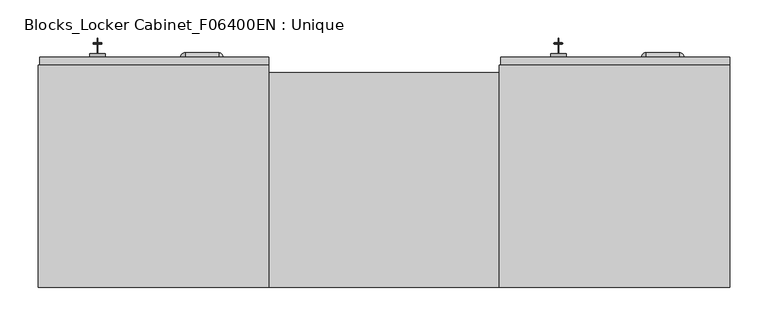
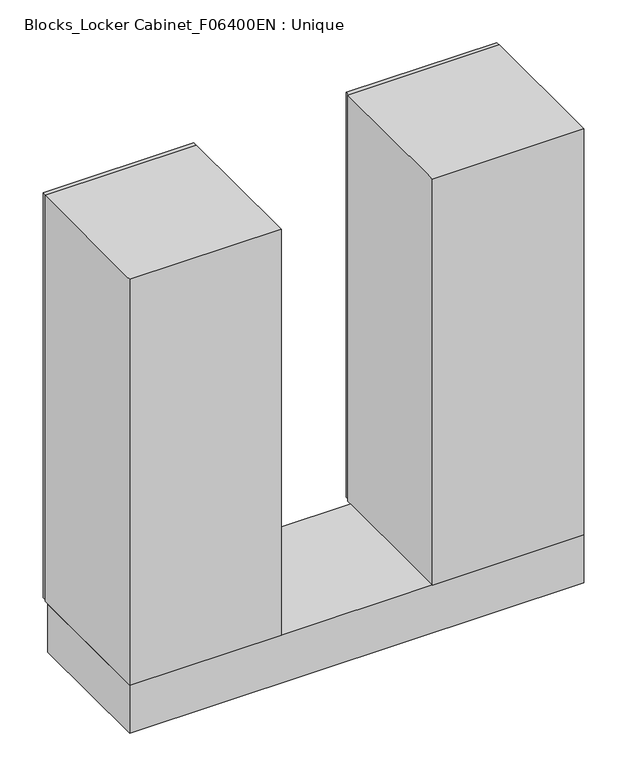
"""IFC4 building model written with IfcOpenShell, lengths in millimetres: furniture geometry, Blocks_Locker Cabinet_F06400EN : Unique."""

from ifc_helpers import new_model, si_unit, point, frame, frame_2d, origin, origin_with_axes, place, context, project, spatial, polyline, circle_curve, ellipse_curve, trimmed, segment, composite_curve, outline, extrude, faceted_brep, source, transform, mapped, element, save
from ifc_brep_helpers import plane_surface, cylinder_surface, revolved_surface, advanced_brep


def blocks_locker_cabinet_f06400en_unique_000e14be(model_context):
    return source(origin(), model_context, "Body", "SolidModel", [
        advanced_brep(
        [(217.0, 12.5, 525.0), (237.0, 12.5, 525.0), (228.8411805, 12.5, 532.0962926), (225.1588195, 12.5, 532.0962926), (225.1588195, 12.5, 522.8618188), (228.8411805, 12.5, 522.8618188), (217.0, 7.5, 525.0), (237.0, 7.5, 525.0), (237.0, 10.7450625, 525.0), (217.0, 10.7450625, 525.0), (228.8411805, 10.7450625, 522.8618188), (228.8411805, 10.7450625, 532.0962926), (225.1588195, 10.7450625, 522.8618188), (225.1588195, 10.7450625, 532.0962926)],
        [
            (0, 1, circle_curve(frame((227.0, 12.5, 525.0), z_axis=(0.0, 1.0, 0.0), x_axis=(1.0, 0.0, 0.0)), 10.0)),
            (1, 0, circle_curve(frame((227.0, 12.5, 525.0), z_axis=(0.0, 1.0, 0.0), x_axis=(1.0, 0.0, 0.0)), 10.0)),
            (2, 3),
            (3, 4),
            (4, 5),
            (5, 2),
            (6, 7, circle_curve(frame((227.0, 7.5, 525.0), z_axis=(0.0, -1.0, 0.0), x_axis=(1.0, 0.0, 0.0)), 10.0)),
            (7, 6, circle_curve(frame((227.0, 7.5, 525.0), z_axis=(0.0, -1.0, 0.0), x_axis=(1.0, 0.0, 0.0)), 10.0)),
            (1, 8),
            (8, 7),
            (6, 9),
            (9, 0),
            (5, 10),
            (10, 11),
            (11, 2),
            (4, 12),
            (12, 10),
            (3, 13),
            (13, 12),
            (11, 13),
        ],
        [
            plane_surface(frame((237.0, 12.5, 525.0), z_axis=(0.0, 1.0, 0.0), x_axis=(0.0, 0.0, 1.0))),
            plane_surface(frame((237.0, 7.5, 525.0), z_axis=(0.0, -1.0, 0.0), x_axis=(0.0, 0.0, -1.0))),
            cylinder_surface(frame((227.0, 7.5, 525.0), z_axis=(0.0, 1.0, 0.0), x_axis=(1.0, 0.0, 0.0)), 10.0),
            plane_surface(frame((228.8411805, 12.5, 532.0962926), z_axis=(-1.0, 0.0, 0.0), x_axis=(0.0, -1.0, 0.0))),
            plane_surface(frame((228.8411805, 12.5, 522.8618188), z_axis=(0.0, 0.0, 1.0), x_axis=(0.0, -1.0, 0.0))),
            plane_surface(frame((225.1588195, 12.5, 522.8618188), z_axis=(1.0, 0.0, 0.0), x_axis=(0.0, -1.0, 0.0))),
            plane_surface(frame((225.1588195, 12.5, 532.0962926), z_axis=(0.0, 0.0, -1.0), x_axis=(0.0, -1.0, 0.0))),
            plane_surface(frame((237.0, 10.7450625, 525.0), z_axis=(0.0, 1.0, 0.0), x_axis=(0.0, 0.0, 1.0))),
        ],
        [
            (0, [[1, 2], [3, 4, 5, 6]]),
            (1, [[7, 8]]),
            (2, [[9, 10, -7, 11, 12, -2]]),
            (2, [[-12, -11, -8, -10, -9, -1]]),
            (3, [[13, 14, 15, -6]]),
            (4, [[16, 17, -13, -5]]),
            (5, [[18, 19, -16, -4]]),
            (6, [[-15, 20, -18, -3]]),
            (7, [[-17, -19, -20, -14]]),
        ],
    ),
        extrude(outline(composite_curve([segment(polyline([(16.8246351, 522.8618188), (13.7848488, 522.8618188)]), True, "CONTINUOUS"), segment(trimmed(circle_curve(frame_2d((12.908516, 522.8618188)), 0.8763328), [point((13.7848488, 522.8618188))], [point((12.0321832, 522.8618188))], True, "CARTESIAN"), True, "CONTINUOUS"), segment(polyline([(12.0321832, 522.8618188), (10.7450625, 522.8618188), (10.7450625, 527.6669902), (17.0336838, 527.6669902)]), True, "CONTINUOUS"), segment(trimmed(circle_curve(frame_2d((23.0067332, 525.0)), 6.5414185), [point((17.0336838, 527.6669902))], [point((16.8246351, 522.8618188))], False, "CARTESIAN"), True, "CONTINUOUS")], self_intersect=False), holes=[composite_curve([segment(trimmed(circle_curve(frame_2d((25.6281997, 525.0)), 1.688217), [point((27.3164167, 525.0))], [point((23.9399827, 525.0))], True, "CARTESIAN"), True, "CONTINUOUS"), segment(trimmed(circle_curve(frame_2d((25.6281997, 525.0)), 1.688217), [point((23.9399827, 525.0))], [point((27.3164167, 525.0))], True, "CARTESIAN"), True, "CONTINUOUS")], self_intersect=False)]), frame((226.5956922, 0.0, 0.0), z_axis=(1.0, 0.0, 0.0), x_axis=(0.0, 1.0, 0.0)), (0.0, 0.0, 1.0), 0.9157402),
        extrude(outline(composite_curve([segment(polyline([(27.8125, 504.8018875), (27.8125, 501.7621012)]), True, "CONTINUOUS"), segment(trimmed(circle_curve(frame_2d((27.8125, 500.8857684)), 0.8763328), [point((27.8125, 501.7621012))], [point((27.8125, 500.0094356))], True, "CARTESIAN"), True, "CONTINUOUS"), segment(polyline([(27.8125, 500.0094356), (27.8125, 497.7621012)]), True, "CONTINUOUS"), segment(trimmed(circle_curve(frame_2d((27.8125, 496.8857684)), 0.8763328), [point((27.8125, 497.7621012))], [point((27.8125, 496.0094356))], True, "CARTESIAN"), True, "CONTINUOUS"), segment(polyline([(27.8125, 496.0094356), (27.8125, 493.7621012)]), True, "CONTINUOUS"), segment(trimmed(circle_curve(frame_2d((27.8125, 492.8857684)), 0.8763328), [point((27.8125, 493.7621012))], [point((27.8125, 492.0094356))], True, "CARTESIAN"), True, "CONTINUOUS"), segment(polyline([(27.8125, 492.0094356), (27.8125, 490.3532579), (25.9613419, 487.7095301), (24.2573286, 487.7095301), (24.2573286, 504.5978839)]), True, "CONTINUOUS"), segment(trimmed(circle_curve(frame_2d((25.6743188, 510.9839856)), 6.5414185), [point((24.2573286, 504.5978839))], [point((27.8125, 504.8018875))], False, "CARTESIAN"), True, "CONTINUOUS")], self_intersect=False), holes=[composite_curve([segment(trimmed(circle_curve(frame_2d((25.6743188, 513.6054521)), 1.688217), [point((25.6743188, 515.2936691))], [point((25.6743188, 511.9172351))], True, "CARTESIAN"), True, "CONTINUOUS"), segment(trimmed(circle_curve(frame_2d((25.6743188, 513.6054521)), 1.688217), [point((25.6743188, 511.9172351))], [point((25.6743188, 515.2936691))], True, "CARTESIAN"), True, "CONTINUOUS")], self_intersect=False)]), frame((226.5956922, 0.0, 0.0), z_axis=(1.0, 0.0, 0.0), x_axis=(0.0, 1.0, 0.0)), (0.0, 0.0, 1.0), 0.9157402),
        advanced_brep(
        [(231.2, 25.663019, 519.4000012), (232.8, 25.663019, 519.4000012), (221.2, 25.663019, 519.4000012), (222.8, 25.663019, 519.4000012)],
        [
            (0, 1, circle_curve(frame((232.0, 25.663019, 519.4000012), z_axis=(0.0, 0.0, -1.0), x_axis=(-1.0, 0.0, 0.0)), 0.8)),
            (1, 2, circle_curve(frame((227.0, 25.663019, 519.4000012), z_axis=(0.0, 1.0, 0.0), x_axis=(-1.0, 0.0, 0.0)), 5.8)),
            (2, 3, circle_curve(frame((222.0, 25.663019, 519.4000012), z_axis=(0.0, 0.0, -1.0), x_axis=(1.0, 0.0, 0.0)), 0.8)),
            (3, 0, circle_curve(frame((227.0, 25.663019, 519.4000012), z_axis=(0.0, -1.0, 0.0), x_axis=(-1.0, 0.0, 0.0)), 4.2)),
            (1, 0, circle_curve(frame((232.0, 25.663019, 519.4000012), z_axis=(0.0, 0.0, -1.0), x_axis=(-1.0, 0.0, 0.0)), 0.8)),
            (3, 2, circle_curve(frame((222.0, 25.663019, 519.4000012), z_axis=(0.0, 0.0, -1.0), x_axis=(1.0, 0.0, 0.0)), 0.8)),
            (2, 1, circle_curve(frame((227.0, 25.663019, 519.4000012), z_axis=(0.0, 1.0, 0.0), x_axis=(1.0, 0.0, 0.0)), 5.8)),
            (0, 3, circle_curve(frame((227.0, 25.663019, 519.4000012), z_axis=(0.0, -1.0, 0.0), x_axis=(1.0, 0.0, 0.0)), 4.2)),
        ],
        [
            revolved_surface(trimmed(ellipse_curve(frame((222.0, 25.663019, 519.4000012), z_axis=(0.0, 0.0, -1.0), x_axis=(1.0, 0.0, 0.0)), 0.8, 0.8), [point((221.2, 25.663019, 519.4000012))], [point((222.8, 25.663019, 519.4000012))], True, "CARTESIAN"), (227.0, -2.5, 519.4000012), (0.0, 1.0, 0.0)),
            revolved_surface(trimmed(ellipse_curve(frame((222.0, 25.663019, 519.4000012), z_axis=(0.0, 0.0, -1.0), x_axis=(1.0, 0.0, 0.0)), 0.8, 0.8), [point((222.8, 25.663019, 519.4000012))], [point((221.2, 25.663019, 519.4000012))], True, "CARTESIAN"), (227.0, -2.5, 519.4000012), (0.0, 1.0, 0.0)),
            revolved_surface(trimmed(ellipse_curve(frame((232.0, 25.663019, 519.4000012), z_axis=(0.0, 0.0, 1.0), x_axis=(-1.0, 0.0, 0.0)), 0.8, 0.8), [point((232.8, 25.663019, 519.4000012))], [point((231.2, 25.663019, 519.4000012))], True, "CARTESIAN"), (227.0, -2.5, 519.4000012), (0.0, 1.0, 0.0)),
            revolved_surface(trimmed(ellipse_curve(frame((232.0, 25.663019, 519.4000012), z_axis=(0.0, 0.0, 1.0), x_axis=(-1.0, 0.0, 0.0)), 0.8, 0.8), [point((231.2, 25.663019, 519.4000012))], [point((232.8, 25.663019, 519.4000012))], True, "CARTESIAN"), (227.0, -2.5, 519.4000012), (0.0, 1.0, 0.0)),
        ],
        [
            (0, [[1, 2, 3, 4]]),
            (1, [[5, -4, 6, -2]]),
            (2, [[-3, 7, -1, 8]]),
            (3, [[-6, -8, -5, -7]]),
        ],
    ),
        advanced_brep(
        [(152.0, 7.5, 949.0), (152.0, -2.5, 949.0), (450.0, -2.5, 949.0), (450.0, 7.5, 949.0), (152.0, 7.5, 101.0), (450.0, 7.5, 101.0), (450.0, -2.5, 101.0), (152.0, -2.5, 101.0), (207.0, 7.5, 675.0), (207.0, 7.5, 555.0), (266.2109264, 7.5, 555.0), (266.2109264, 7.5, 675.0), (219.3473099, 0.3712773, 675.0), (242.7894451, 3.975278, 675.0), (219.3473099, 0.3712773, 555.0), (242.7894451, 3.975278, 555.0)],
        [
            (0, 1),
            (1, 2),
            (2, 3),
            (3, 0),
            (4, 5),
            (5, 6),
            (6, 7),
            (7, 4),
            (3, 5),
            (4, 0),
            (8, 9),
            (9, 10),
            (10, 11),
            (11, 8),
            (2, 6),
            (1, 7),
            (12, 8),
            (11, 13),
            (13, 12, circle_curve(frame((228.8223477, 16.7825242, 675.0), z_axis=(0.0, 0.0, -1.0), x_axis=(0.0, 1.0, 0.0)), 18.9500756)),
            (14, 15, circle_curve(frame((228.8223477, 16.7825242, 555.0), z_axis=(0.0, 0.0, 1.0), x_axis=(0.0, 1.0, 0.0)), 18.9500756)),
            (15, 10),
            (9, 14),
            (12, 14),
            (15, 13),
        ],
        [
            plane_surface(frame((450.0, 7.5, 949.0), z_axis=(0.0, 0.0, 1.0), x_axis=(1.0, 0.0, 0.0))),
            plane_surface(frame((450.0, 7.5, 101.0), z_axis=(0.0, 0.0, -1.0), x_axis=(-1.0, 0.0, 0.0))),
            plane_surface(frame((152.0, 7.5, 949.0), z_axis=(0.0, 1.0, 0.0), x_axis=(0.0, 0.0, -1.0))),
            plane_surface(frame((450.0, 7.5, 949.0), z_axis=(1.0, 0.0, 0.0), x_axis=(0.0, 0.0, -1.0))),
            plane_surface(frame((450.0, -2.5, 949.0), z_axis=(0.0, -1.0, 0.0), x_axis=(0.0, 0.0, -1.0))),
            plane_surface(frame((152.0, -2.5, 949.0), z_axis=(-1.0, 0.0, 0.0), x_axis=(0.0, 0.0, -1.0))),
            plane_surface(frame((207.0, 7.5, 675.0), z_axis=(0.0, 0.0, -1.0), x_axis=(-0.866025403784437, 0.5000000000000028, 0.0))),
            plane_surface(frame((207.0, 7.5, 555.0), z_axis=(0.0, 0.0, 1.0), x_axis=(0.866025403784437, -0.5000000000000028, 0.0))),
            plane_surface(frame((219.3473099, 0.3712773, 675.0), z_axis=(0.5000000000000028, 0.866025403784437, 0.0), x_axis=(0.0, 0.0, -1.0))),
            plane_surface(frame((266.2109264, 7.5, 675.0), z_axis=(-0.14881527984319862, 0.9888650122666847, 0.0), x_axis=(0.0, 0.0, -1.0))),
            revolved_surface(polyline([(228.8223477, 35.7325998, 675.0), (228.8223477, 35.7325998, 555.0)]), (228.8223477, 16.7825242, 555.0), (0.0, 0.0, 1.0)),
        ],
        [
            (0, [[1, 2, 3, 4]]),
            (1, [[5, 6, 7, 8]]),
            (2, [[9, -5, 10, -4], [11, 12, 13, 14]]),
            (3, [[15, -6, -9, -3]]),
            (4, [[16, -7, -15, -2]]),
            (5, [[-10, -8, -16, -1]]),
            (6, [[17, -14, 18, 19]]),
            (7, [[20, 21, -12, 22]]),
            (8, [[23, -22, -11, -17]]),
            (9, [[-13, -21, 24, -18]]),
            (10, [[-24, -20, -23, -19]]),
        ],
    ),
        advanced_brep(
        [(335.0, 7.5, 141.0), (390.5189667, 7.5, 141.0), (384.5189667, 7.5, 147.0), (341.0, 7.5, 147.0), (341.0, 13.5, 141.0), (384.5189667, 13.5, 141.0)],
        [
            (0, 1),
            (1, 2, circle_curve(frame((384.5189667, 7.5, 141.0), z_axis=(0.0, -1.0, 0.0), x_axis=(1.0, 0.0, 0.0)), 6.0)),
            (2, 3),
            (3, 0, circle_curve(frame((341.0, 7.5, 141.0), z_axis=(0.0, -1.0, 0.0), x_axis=(1.0, 0.0, 0.0)), 6.0)),
            (0, 4, circle_curve(frame((341.0, 7.5, 141.0), z_axis=(0.0, 0.0, -1.0), x_axis=(1.0, 0.0, 0.0)), 6.0)),
            (4, 5),
            (5, 1, circle_curve(frame((384.5189667, 7.5, 141.0), z_axis=(0.0, 0.0, -1.0), x_axis=(1.0, 0.0, 0.0)), 6.0)),
            (3, 4, circle_curve(frame((341.0, 7.5, 141.0), z_axis=(-1.0, 0.0, 0.0), x_axis=(0.0, 0.0, 1.0)), 6.0)),
            (2, 5, circle_curve(frame((384.5189667, 7.5, 141.0), z_axis=(-1.0, 0.0, 0.0), x_axis=(0.0, 0.0, 1.0)), 6.0)),
        ],
        [
            plane_surface(frame((385.0, 7.5, 141.0), z_axis=(0.0, -1.0, 0.0), x_axis=(0.0, 0.0, 1.0))),
            plane_surface(frame((385.0, 7.5, 141.0), z_axis=(0.0, 0.0, -1.0), x_axis=(0.0, 1.0, 0.0))),
            revolved_surface(trimmed(ellipse_curve(frame((341.0, 7.5, 141.0), z_axis=(0.0, 1.0, 0.0), x_axis=(1.0, 0.0, 0.0)), 6.0, 6.0), [point((335.0, 7.5, 141.0))], [point((341.0, 7.5, 147.0))], True, "CARTESIAN"), (385.0, 7.5, 141.0), (1.0, 0.0, 0.0)),
            cylinder_surface(frame((385.0, 7.5, 141.0), z_axis=(1.0, 0.0, 0.0), x_axis=(0.0, 0.0, 1.0)), 6.0),
            revolved_surface(trimmed(ellipse_curve(frame((384.5189667, 7.5, 141.0), z_axis=(0.0, 1.0, 0.0), x_axis=(1.0, 0.0, 0.0)), 6.0, 6.0), [point((384.5189667, 7.5, 147.0))], [point((390.5189667, 7.5, 141.0))], True, "CARTESIAN"), (385.0, 7.5, 141.0), (1.0, 0.0, 0.0)),
        ],
        [
            (0, [[1, 2, 3, 4]]),
            (1, [[-1, 5, 6, 7]]),
            (2, [[-5, -4, 8]]),
            (3, [[-6, -8, -3, 9]]),
            (4, [[-7, -9, -2]]),
        ],
    ),
        advanced_brep(
        [(335.0, 7.5, 156.0), (390.5189667, 7.5, 156.0), (384.5189667, 7.5, 162.0), (341.0, 7.5, 162.0), (341.0, 13.5, 156.0), (384.5189667, 13.5, 156.0)],
        [
            (0, 1),
            (1, 2, circle_curve(frame((384.5189667, 7.5, 156.0), z_axis=(0.0, -1.0, 0.0), x_axis=(1.0, 0.0, 0.0)), 6.0)),
            (2, 3),
            (3, 0, circle_curve(frame((341.0, 7.5, 156.0), z_axis=(0.0, -1.0, 0.0), x_axis=(1.0, 0.0, 0.0)), 6.0)),
            (0, 4, circle_curve(frame((341.0, 7.5, 156.0), z_axis=(0.0, 0.0, -1.0), x_axis=(1.0, 0.0, 0.0)), 6.0)),
            (4, 5),
            (5, 1, circle_curve(frame((384.5189667, 7.5, 156.0), z_axis=(0.0, 0.0, -1.0), x_axis=(1.0, 0.0, 0.0)), 6.0)),
            (3, 4, circle_curve(frame((341.0, 7.5, 156.0), z_axis=(-1.0, 0.0, 0.0), x_axis=(0.0, 0.0, 1.0)), 6.0)),
            (2, 5, circle_curve(frame((384.5189667, 7.5, 156.0), z_axis=(-1.0, 0.0, 0.0), x_axis=(0.0, 0.0, 1.0)), 6.0)),
        ],
        [
            plane_surface(frame((385.0, 7.5, 156.0), z_axis=(0.0, -1.0, 0.0), x_axis=(0.0, 0.0, 1.0))),
            plane_surface(frame((385.0, 7.5, 156.0), z_axis=(0.0, 0.0, -1.0), x_axis=(0.0, 1.0, 0.0))),
            revolved_surface(trimmed(ellipse_curve(frame((341.0, 7.5, 156.0), z_axis=(0.0, 1.0, 0.0), x_axis=(1.0, 0.0, 0.0)), 6.0, 6.0), [point((335.0, 7.5, 156.0))], [point((341.0, 7.5, 162.0))], True, "CARTESIAN"), (385.0, 7.5, 156.0), (1.0, 0.0, 0.0)),
            cylinder_surface(frame((385.0, 7.5, 156.0), z_axis=(1.0, 0.0, 0.0), x_axis=(0.0, 0.0, 1.0)), 6.0),
            revolved_surface(trimmed(ellipse_curve(frame((384.5189667, 7.5, 156.0), z_axis=(0.0, 1.0, 0.0), x_axis=(1.0, 0.0, 0.0)), 6.0, 6.0), [point((384.5189667, 7.5, 162.0))], [point((390.5189667, 7.5, 156.0))], True, "CARTESIAN"), (385.0, 7.5, 156.0), (1.0, 0.0, 0.0)),
        ],
        [
            (0, [[1, 2, 3, 4]]),
            (1, [[-1, 5, 6, 7]]),
            (2, [[-5, -4, 8]]),
            (3, [[-6, -8, -3, 9]]),
            (4, [[-7, -9, -2]]),
        ],
    ),
        advanced_brep(
        [(335.0, 7.5, 171.0), (390.5189667, 7.5, 171.0), (384.5189667, 7.5, 177.0), (341.0, 7.5, 177.0), (341.0, 13.5, 171.0), (384.5189667, 13.5, 171.0)],
        [
            (0, 1),
            (1, 2, circle_curve(frame((384.5189667, 7.5, 171.0), z_axis=(0.0, -1.0, 0.0), x_axis=(1.0, 0.0, 0.0)), 6.0)),
            (2, 3),
            (3, 0, circle_curve(frame((341.0, 7.5, 171.0), z_axis=(0.0, -1.0, 0.0), x_axis=(1.0, 0.0, 0.0)), 6.0)),
            (0, 4, circle_curve(frame((341.0, 7.5, 171.0), z_axis=(0.0, 0.0, -1.0), x_axis=(1.0, 0.0, 0.0)), 6.0)),
            (4, 5),
            (5, 1, circle_curve(frame((384.5189667, 7.5, 171.0), z_axis=(0.0, 0.0, -1.0), x_axis=(1.0, 0.0, 0.0)), 6.0)),
            (3, 4, circle_curve(frame((341.0, 7.5, 171.0), z_axis=(-1.0, 0.0, 0.0), x_axis=(0.0, 0.0, 1.0)), 6.0)),
            (2, 5, circle_curve(frame((384.5189667, 7.5, 171.0), z_axis=(-1.0, 0.0, 0.0), x_axis=(0.0, 0.0, 1.0)), 6.0)),
        ],
        [
            plane_surface(frame((385.0, 7.5, 171.0), z_axis=(0.0, -1.0, 0.0), x_axis=(0.0, 0.0, 1.0))),
            plane_surface(frame((385.0, 7.5, 171.0), z_axis=(0.0, 0.0, -1.0), x_axis=(0.0, 1.0, 0.0))),
            revolved_surface(trimmed(ellipse_curve(frame((341.0, 7.5, 171.0), z_axis=(0.0, 1.0, 0.0), x_axis=(1.0, 0.0, 0.0)), 6.0, 6.0), [point((335.0, 7.5, 171.0))], [point((341.0, 7.5, 177.0))], True, "CARTESIAN"), (385.0, 7.5, 171.0), (1.0, 0.0, 0.0)),
            cylinder_surface(frame((385.0, 7.5, 171.0), z_axis=(1.0, 0.0, 0.0), x_axis=(0.0, 0.0, 1.0)), 6.0),
            revolved_surface(trimmed(ellipse_curve(frame((384.5189667, 7.5, 171.0), z_axis=(0.0, 1.0, 0.0), x_axis=(1.0, 0.0, 0.0)), 6.0, 6.0), [point((384.5189667, 7.5, 177.0))], [point((390.5189667, 7.5, 171.0))], True, "CARTESIAN"), (385.0, 7.5, 171.0), (1.0, 0.0, 0.0)),
        ],
        [
            (0, [[1, 2, 3, 4]]),
            (1, [[-1, 5, 6, 7]]),
            (2, [[-5, -4, 8]]),
            (3, [[-6, -8, -3, 9]]),
            (4, [[-7, -9, -2]]),
        ],
    ),
        advanced_brep(
        [(335.0, 7.5, 186.0), (390.5189667, 7.5, 186.0), (384.5189667, 7.5, 192.0), (341.0, 7.5, 192.0), (341.0, 13.5, 186.0), (384.5189667, 13.5, 186.0)],
        [
            (0, 1),
            (1, 2, circle_curve(frame((384.5189667, 7.5, 186.0), z_axis=(0.0, -1.0, 0.0), x_axis=(1.0, 0.0, 0.0)), 6.0)),
            (2, 3),
            (3, 0, circle_curve(frame((341.0, 7.5, 186.0), z_axis=(0.0, -1.0, 0.0), x_axis=(1.0, 0.0, 0.0)), 6.0)),
            (0, 4, circle_curve(frame((341.0, 7.5, 186.0), z_axis=(0.0, 0.0, -1.0), x_axis=(1.0, 0.0, 0.0)), 6.0)),
            (4, 5),
            (5, 1, circle_curve(frame((384.5189667, 7.5, 186.0), z_axis=(0.0, 0.0, -1.0), x_axis=(1.0, 0.0, 0.0)), 6.0)),
            (3, 4, circle_curve(frame((341.0, 7.5, 186.0), z_axis=(-1.0, 0.0, 0.0), x_axis=(0.0, 0.0, 1.0)), 6.0)),
            (2, 5, circle_curve(frame((384.5189667, 7.5, 186.0), z_axis=(-1.0, 0.0, 0.0), x_axis=(0.0, 0.0, 1.0)), 6.0)),
        ],
        [
            plane_surface(frame((385.0, 7.5, 186.0), z_axis=(0.0, -1.0, 0.0), x_axis=(0.0, 0.0, 1.0))),
            plane_surface(frame((385.0, 7.5, 186.0), z_axis=(0.0, 0.0, -1.0), x_axis=(0.0, 1.0, 0.0))),
            revolved_surface(trimmed(ellipse_curve(frame((341.0, 7.5, 186.0), z_axis=(0.0, 1.0, 0.0), x_axis=(1.0, 0.0, 0.0)), 6.0, 6.0), [point((335.0, 7.5, 186.0))], [point((341.0, 7.5, 192.0))], True, "CARTESIAN"), (385.0, 7.5, 186.0), (1.0, 0.0, 0.0)),
            cylinder_surface(frame((385.0, 7.5, 186.0), z_axis=(1.0, 0.0, 0.0), x_axis=(0.0, 0.0, 1.0)), 6.0),
            revolved_surface(trimmed(ellipse_curve(frame((384.5189667, 7.5, 186.0), z_axis=(0.0, 1.0, 0.0), x_axis=(1.0, 0.0, 0.0)), 6.0, 6.0), [point((384.5189667, 7.5, 192.0))], [point((390.5189667, 7.5, 186.0))], True, "CARTESIAN"), (385.0, 7.5, 186.0), (1.0, 0.0, 0.0)),
        ],
        [
            (0, [[1, 2, 3, 4]]),
            (1, [[-1, 5, 6, 7]]),
            (2, [[-5, -4, 8]]),
            (3, [[-6, -8, -3, 9]]),
            (4, [[-7, -9, -2]]),
        ],
    ),
        advanced_brep(
        [(335.0, 7.5, 201.0), (390.5189667, 7.5, 201.0), (384.5189667, 7.5, 207.0), (341.0, 7.5, 207.0), (341.0, 13.5, 201.0), (384.5189667, 13.5, 201.0)],
        [
            (0, 1),
            (1, 2, circle_curve(frame((384.5189667, 7.5, 201.0), z_axis=(0.0, -1.0, 0.0), x_axis=(1.0, 0.0, 0.0)), 6.0)),
            (2, 3),
            (3, 0, circle_curve(frame((341.0, 7.5, 201.0), z_axis=(0.0, -1.0, 0.0), x_axis=(1.0, 0.0, 0.0)), 6.0)),
            (0, 4, circle_curve(frame((341.0, 7.5, 201.0), z_axis=(0.0, 0.0, -1.0), x_axis=(1.0, 0.0, 0.0)), 6.0)),
            (4, 5),
            (5, 1, circle_curve(frame((384.5189667, 7.5, 201.0), z_axis=(0.0, 0.0, -1.0), x_axis=(1.0, 0.0, 0.0)), 6.0)),
            (3, 4, circle_curve(frame((341.0, 7.5, 201.0), z_axis=(-1.0, 0.0, 0.0), x_axis=(0.0, 0.0, 1.0)), 6.0)),
            (2, 5, circle_curve(frame((384.5189667, 7.5, 201.0), z_axis=(-1.0, 0.0, 0.0), x_axis=(0.0, 0.0, 1.0)), 6.0)),
        ],
        [
            plane_surface(frame((385.0, 7.5, 201.0), z_axis=(0.0, -1.0, 0.0), x_axis=(0.0, 0.0, 1.0))),
            plane_surface(frame((385.0, 7.5, 201.0), z_axis=(0.0, 0.0, -1.0), x_axis=(0.0, 1.0, 0.0))),
            revolved_surface(trimmed(ellipse_curve(frame((341.0, 7.5, 201.0), z_axis=(0.0, 1.0, 0.0), x_axis=(1.0, 0.0, 0.0)), 6.0, 6.0), [point((335.0, 7.5, 201.0))], [point((341.0, 7.5, 207.0))], True, "CARTESIAN"), (385.0, 7.5, 201.0), (1.0, 0.0, 0.0)),
            cylinder_surface(frame((385.0, 7.5, 201.0), z_axis=(1.0, 0.0, 0.0), x_axis=(0.0, 0.0, 1.0)), 6.0),
            revolved_surface(trimmed(ellipse_curve(frame((384.5189667, 7.5, 201.0), z_axis=(0.0, 1.0, 0.0), x_axis=(1.0, 0.0, 0.0)), 6.0, 6.0), [point((384.5189667, 7.5, 207.0))], [point((390.5189667, 7.5, 201.0))], True, "CARTESIAN"), (385.0, 7.5, 201.0), (1.0, 0.0, 0.0)),
        ],
        [
            (0, [[1, 2, 3, 4]]),
            (1, [[-1, 5, 6, 7]]),
            (2, [[-5, -4, 8]]),
            (3, [[-6, -8, -3, 9]]),
            (4, [[-7, -9, -2]]),
        ],
    ),
        extrude(outline(composite_curve([segment(polyline([(219.3473099, 0.3712773), (207.0, 7.5), (266.2109264, 7.5), (242.7894451, 3.975278)]), True, "CONTINUOUS"), segment(trimmed(circle_curve(frame_2d((228.8223477, 16.7825242)), 18.9500756), [point((242.7894451, 3.975278))], [point((219.3473099, 0.3712773))], False, "CARTESIAN"), True, "CONTINUOUS")], self_intersect=False)), frame((0.0, 0.0, 555.0), z_axis=(0.0, 0.0, 1.0), x_axis=(1.0, 0.0, 0.0)), (0.0, 0.0, 1.0), 5.0),
        extrude(outline(composite_curve([segment(polyline([(219.3473099, 0.3712773), (207.0, 7.5), (266.2109264, 7.5), (242.7894451, 3.975278)]), True, "CONTINUOUS"), segment(trimmed(circle_curve(frame_2d((228.8223477, 16.7825242)), 18.9500756), [point((242.7894451, 3.975278))], [point((219.3473099, 0.3712773))], False, "CARTESIAN"), True, "CONTINUOUS")], self_intersect=False)), frame((0.0, 0.0, 670.0), z_axis=(0.0, 0.0, 1.0), x_axis=(1.0, 0.0, 0.0)), (0.0, 0.0, 1.0), 5.0),
        faceted_brep([(450.0, -2.5, 950.0), (450.0, -2.5, 100.0), (150.0, -2.5, 100.0), (150.0, -2.5, 950.0), (440.0, -2.5, 940.0), (160.0, -2.5, 940.0), (160.0, -2.5, 110.0), (440.0, -2.5, 110.0), (450.0, -292.5, 950.0), (150.0, -292.5, 950.0), (150.0, -292.5, 100.0), (450.0, -292.5, 100.0), (150.0, -282.5, 950.0), (450.0, -282.5, 950.0), (150.0, -282.5, 100.0), (450.0, -282.5, 100.0), (440.0, -282.5, 110.0), (440.0, -282.5, 940.0), (160.0, -282.5, 110.0), (160.0, -282.5, 940.0)], [[[0, 1, 2, 3], [4, 5, 6, 7]], [[8, 9, 10, 11]], [[3, 12, 9, 8, 13, 0]], [[2, 14, 10, 9, 12, 3]], [[1, 15, 11, 10, 14, 2]], [[0, 13, 8, 11, 15, 1]], [[7, 16, 17, 4]], [[6, 18, 16, 7]], [[5, 19, 18, 6]], [[4, 17, 19, 5]], [[16, 18, 19, 17]]]),
        advanced_brep(
        [(-383.0, 12.5, 525.0), (-363.0, 12.5, 525.0), (-371.1588195, 12.5, 532.0962926), (-374.8411805, 12.5, 532.0962926), (-374.8411805, 12.5, 522.8618188), (-371.1588195, 12.5, 522.8618188), (-383.0, 7.5, 525.0), (-363.0, 7.5, 525.0), (-363.0, 10.7450625, 525.0), (-383.0, 10.7450625, 525.0), (-371.1588195, 10.7450625, 522.8618188), (-371.1588195, 10.7450625, 532.0962926), (-374.8411805, 10.7450625, 522.8618188), (-374.8411805, 10.7450625, 532.0962926)],
        [
            (0, 1, circle_curve(frame((-373.0, 12.5, 525.0), z_axis=(0.0, 1.0, 0.0), x_axis=(1.0, 0.0, 0.0)), 10.0)),
            (1, 0, circle_curve(frame((-373.0, 12.5, 525.0), z_axis=(0.0, 1.0, 0.0), x_axis=(1.0, 0.0, 0.0)), 10.0)),
            (2, 3),
            (3, 4),
            (4, 5),
            (5, 2),
            (6, 7, circle_curve(frame((-373.0, 7.5, 525.0), z_axis=(0.0, -1.0, 0.0), x_axis=(1.0, 0.0, 0.0)), 10.0)),
            (7, 6, circle_curve(frame((-373.0, 7.5, 525.0), z_axis=(0.0, -1.0, 0.0), x_axis=(1.0, 0.0, 0.0)), 10.0)),
            (1, 8),
            (8, 7),
            (6, 9),
            (9, 0),
            (5, 10),
            (10, 11),
            (11, 2),
            (4, 12),
            (12, 10),
            (3, 13),
            (13, 12),
            (11, 13),
        ],
        [
            plane_surface(frame((-363.0, 12.5, 525.0), z_axis=(0.0, 1.0, 0.0), x_axis=(0.0, 0.0, 1.0))),
            plane_surface(frame((-363.0, 7.5, 525.0), z_axis=(0.0, -1.0, 0.0), x_axis=(0.0, 0.0, -1.0))),
            cylinder_surface(frame((-373.0, 7.5, 525.0), z_axis=(0.0, 1.0, 0.0), x_axis=(1.0, 0.0, 0.0)), 10.0),
            plane_surface(frame((-371.1588195, 12.5, 532.0962926), z_axis=(-1.0, 0.0, 0.0), x_axis=(0.0, -1.0, 0.0))),
            plane_surface(frame((-371.1588195, 12.5, 522.8618188), z_axis=(0.0, 0.0, 1.0), x_axis=(0.0, -1.0, 0.0))),
            plane_surface(frame((-374.8411805, 12.5, 522.8618188), z_axis=(1.0, 0.0, 0.0), x_axis=(0.0, -1.0, 0.0))),
            plane_surface(frame((-374.8411805, 12.5, 532.0962926), z_axis=(0.0, 0.0, -1.0), x_axis=(0.0, -1.0, 0.0))),
            plane_surface(frame((-363.0, 10.7450625, 525.0), z_axis=(0.0, 1.0, 0.0), x_axis=(0.0, 0.0, 1.0))),
        ],
        [
            (0, [[1, 2], [3, 4, 5, 6]]),
            (1, [[7, 8]]),
            (2, [[9, 10, -7, 11, 12, -2]]),
            (2, [[-12, -11, -8, -10, -9, -1]]),
            (3, [[13, 14, 15, -6]]),
            (4, [[16, 17, -13, -5]]),
            (5, [[18, 19, -16, -4]]),
            (6, [[-15, 20, -18, -3]]),
            (7, [[-17, -19, -20, -14]]),
        ],
    ),
        extrude(outline(composite_curve([segment(polyline([(16.8246351, 522.8618188), (13.7848488, 522.8618188)]), True, "CONTINUOUS"), segment(trimmed(circle_curve(frame_2d((12.908516, 522.8618188)), 0.8763328), [point((13.7848488, 522.8618188))], [point((12.0321832, 522.8618188))], True, "CARTESIAN"), True, "CONTINUOUS"), segment(polyline([(12.0321832, 522.8618188), (10.7450625, 522.8618188), (10.7450625, 527.6669902), (17.0336838, 527.6669902)]), True, "CONTINUOUS"), segment(trimmed(circle_curve(frame_2d((23.0067332, 525.0)), 6.5414185), [point((17.0336838, 527.6669902))], [point((16.8246351, 522.8618188))], False, "CARTESIAN"), True, "CONTINUOUS")], self_intersect=False), holes=[composite_curve([segment(trimmed(circle_curve(frame_2d((25.6281997, 525.0)), 1.688217), [point((27.3164167, 525.0))], [point((23.9399827, 525.0))], True, "CARTESIAN"), True, "CONTINUOUS"), segment(trimmed(circle_curve(frame_2d((25.6281997, 525.0)), 1.688217), [point((23.9399827, 525.0))], [point((27.3164167, 525.0))], True, "CARTESIAN"), True, "CONTINUOUS")], self_intersect=False)]), frame((-373.4043078, 0.0, 0.0), z_axis=(1.0, 0.0, 0.0), x_axis=(0.0, 1.0, 0.0)), (0.0, 0.0, 1.0), 0.9157402),
        extrude(outline(composite_curve([segment(polyline([(27.8125, 504.8018875), (27.8125, 501.7621012)]), True, "CONTINUOUS"), segment(trimmed(circle_curve(frame_2d((27.8125, 500.8857684)), 0.8763328), [point((27.8125, 501.7621012))], [point((27.8125, 500.0094356))], True, "CARTESIAN"), True, "CONTINUOUS"), segment(polyline([(27.8125, 500.0094356), (27.8125, 497.7621012)]), True, "CONTINUOUS"), segment(trimmed(circle_curve(frame_2d((27.8125, 496.8857684)), 0.8763328), [point((27.8125, 497.7621012))], [point((27.8125, 496.0094356))], True, "CARTESIAN"), True, "CONTINUOUS"), segment(polyline([(27.8125, 496.0094356), (27.8125, 493.7621012)]), True, "CONTINUOUS"), segment(trimmed(circle_curve(frame_2d((27.8125, 492.8857684)), 0.8763328), [point((27.8125, 493.7621012))], [point((27.8125, 492.0094356))], True, "CARTESIAN"), True, "CONTINUOUS"), segment(polyline([(27.8125, 492.0094356), (27.8125, 490.3532579), (25.9613419, 487.7095301), (24.2573286, 487.7095301), (24.2573286, 504.5978839)]), True, "CONTINUOUS"), segment(trimmed(circle_curve(frame_2d((25.6743188, 510.9839856)), 6.5414185), [point((24.2573286, 504.5978839))], [point((27.8125, 504.8018875))], False, "CARTESIAN"), True, "CONTINUOUS")], self_intersect=False), holes=[composite_curve([segment(trimmed(circle_curve(frame_2d((25.6743188, 513.6054521)), 1.688217), [point((25.6743188, 515.2936691))], [point((25.6743188, 511.9172351))], True, "CARTESIAN"), True, "CONTINUOUS"), segment(trimmed(circle_curve(frame_2d((25.6743188, 513.6054521)), 1.688217), [point((25.6743188, 511.9172351))], [point((25.6743188, 515.2936691))], True, "CARTESIAN"), True, "CONTINUOUS")], self_intersect=False)]), frame((-373.4043078, 0.0, 0.0), z_axis=(1.0, 0.0, 0.0), x_axis=(0.0, 1.0, 0.0)), (0.0, 0.0, 1.0), 0.9157402),
        advanced_brep(
        [(-368.8, 25.663019, 519.4000012), (-367.2, 25.663019, 519.4000012), (-378.8, 25.663019, 519.4000012), (-377.2, 25.663019, 519.4000012)],
        [
            (0, 1, circle_curve(frame((-368.0, 25.663019, 519.4000012), z_axis=(0.0, 0.0, -1.0), x_axis=(-1.0, 0.0, 0.0)), 0.8)),
            (1, 2, circle_curve(frame((-373.0, 25.663019, 519.4000012), z_axis=(0.0, 1.0, 0.0), x_axis=(-1.0, 0.0, 0.0)), 5.8)),
            (2, 3, circle_curve(frame((-378.0, 25.663019, 519.4000012), z_axis=(0.0, 0.0, -1.0), x_axis=(1.0, 0.0, 0.0)), 0.8)),
            (3, 0, circle_curve(frame((-373.0, 25.663019, 519.4000012), z_axis=(0.0, -1.0, 0.0), x_axis=(-1.0, 0.0, 0.0)), 4.2)),
            (1, 0, circle_curve(frame((-368.0, 25.663019, 519.4000012), z_axis=(0.0, 0.0, -1.0), x_axis=(-1.0, 0.0, 0.0)), 0.8)),
            (3, 2, circle_curve(frame((-378.0, 25.663019, 519.4000012), z_axis=(0.0, 0.0, -1.0), x_axis=(1.0, 0.0, 0.0)), 0.8)),
            (2, 1, circle_curve(frame((-373.0, 25.663019, 519.4000012), z_axis=(0.0, 1.0, 0.0), x_axis=(1.0, 0.0, 0.0)), 5.8)),
            (0, 3, circle_curve(frame((-373.0, 25.663019, 519.4000012), z_axis=(0.0, -1.0, 0.0), x_axis=(1.0, 0.0, 0.0)), 4.2)),
        ],
        [
            revolved_surface(trimmed(ellipse_curve(frame((-378.0, 25.663019, 519.4000012), z_axis=(0.0, 0.0, -1.0), x_axis=(1.0, 0.0, 0.0)), 0.8, 0.8), [point((-378.8, 25.663019, 519.4000012))], [point((-377.2, 25.663019, 519.4000012))], True, "CARTESIAN"), (-373.0, -2.5, 519.4000012), (0.0, 1.0, 0.0)),
            revolved_surface(trimmed(ellipse_curve(frame((-378.0, 25.663019, 519.4000012), z_axis=(0.0, 0.0, -1.0), x_axis=(1.0, 0.0, 0.0)), 0.8, 0.8), [point((-377.2, 25.663019, 519.4000012))], [point((-378.8, 25.663019, 519.4000012))], True, "CARTESIAN"), (-373.0, -2.5, 519.4000012), (0.0, 1.0, 0.0)),
            revolved_surface(trimmed(ellipse_curve(frame((-368.0, 25.663019, 519.4000012), z_axis=(0.0, 0.0, 1.0), x_axis=(-1.0, 0.0, 0.0)), 0.8, 0.8), [point((-367.2, 25.663019, 519.4000012))], [point((-368.8, 25.663019, 519.4000012))], True, "CARTESIAN"), (-373.0, -2.5, 519.4000012), (0.0, 1.0, 0.0)),
            revolved_surface(trimmed(ellipse_curve(frame((-368.0, 25.663019, 519.4000012), z_axis=(0.0, 0.0, 1.0), x_axis=(-1.0, 0.0, 0.0)), 0.8, 0.8), [point((-368.8, 25.663019, 519.4000012))], [point((-367.2, 25.663019, 519.4000012))], True, "CARTESIAN"), (-373.0, -2.5, 519.4000012), (0.0, 1.0, 0.0)),
        ],
        [
            (0, [[1, 2, 3, 4]]),
            (1, [[5, -4, 6, -2]]),
            (2, [[-3, 7, -1, 8]]),
            (3, [[-6, -8, -5, -7]]),
        ],
    ),
        advanced_brep(
        [(-448.0, 7.5, 949.0), (-448.0, -2.5, 949.0), (-150.0, -2.5, 949.0), (-150.0, 7.5, 949.0), (-448.0, 7.5, 101.0), (-150.0, 7.5, 101.0), (-150.0, -2.5, 101.0), (-448.0, -2.5, 101.0), (-393.0, 7.5, 675.0), (-393.0, 7.5, 555.0), (-333.7890736, 7.5, 555.0), (-333.7890736, 7.5, 675.0), (-380.6526901, 0.3712773, 675.0), (-357.2105549, 3.975278, 675.0), (-380.6526901, 0.3712773, 555.0), (-357.2105549, 3.975278, 555.0)],
        [
            (0, 1),
            (1, 2),
            (2, 3),
            (3, 0),
            (4, 5),
            (5, 6),
            (6, 7),
            (7, 4),
            (3, 5),
            (4, 0),
            (8, 9),
            (9, 10),
            (10, 11),
            (11, 8),
            (2, 6),
            (1, 7),
            (12, 8),
            (11, 13),
            (13, 12, circle_curve(frame((-371.1776523, 16.7825242, 675.0), z_axis=(0.0, 0.0, -1.0), x_axis=(0.0, 1.0, 0.0)), 18.9500756)),
            (14, 15, circle_curve(frame((-371.1776523, 16.7825242, 555.0), z_axis=(0.0, 0.0, 1.0), x_axis=(0.0, 1.0, 0.0)), 18.9500756)),
            (15, 10),
            (9, 14),
            (12, 14),
            (15, 13),
        ],
        [
            plane_surface(frame((-150.0, 7.5, 949.0), z_axis=(0.0, 0.0, 1.0), x_axis=(1.0, 0.0, 0.0))),
            plane_surface(frame((-150.0, 7.5, 101.0), z_axis=(0.0, 0.0, -1.0), x_axis=(-1.0, 0.0, 0.0))),
            plane_surface(frame((-448.0, 7.5, 949.0), z_axis=(0.0, 1.0, 0.0), x_axis=(0.0, 0.0, -1.0))),
            plane_surface(frame((-150.0, 7.5, 949.0), z_axis=(1.0, 0.0, 0.0), x_axis=(0.0, 0.0, -1.0))),
            plane_surface(frame((-150.0, -2.5, 949.0), z_axis=(0.0, -1.0, 0.0), x_axis=(0.0, 0.0, -1.0))),
            plane_surface(frame((-448.0, -2.5, 949.0), z_axis=(-1.0, 0.0, 0.0), x_axis=(0.0, 0.0, -1.0))),
            plane_surface(frame((-393.0, 7.5, 675.0), z_axis=(0.0, 0.0, -1.0), x_axis=(-0.866025403784437, 0.5000000000000028, 0.0))),
            plane_surface(frame((-393.0, 7.5, 555.0), z_axis=(0.0, 0.0, 1.0), x_axis=(0.866025403784437, -0.5000000000000028, 0.0))),
            plane_surface(frame((-380.6526901, 0.3712773, 675.0), z_axis=(0.5000000000000028, 0.866025403784437, 0.0), x_axis=(0.0, 0.0, -1.0))),
            plane_surface(frame((-333.7890736, 7.5, 675.0), z_axis=(-0.14881527984319862, 0.9888650122666847, 0.0), x_axis=(0.0, 0.0, -1.0))),
            revolved_surface(polyline([(-371.1776523, 35.7325998, 675.0), (-371.1776523, 35.7325998, 555.0)]), (-371.1776523, 16.7825242, 555.0), (0.0, 0.0, 1.0)),
        ],
        [
            (0, [[1, 2, 3, 4]]),
            (1, [[5, 6, 7, 8]]),
            (2, [[9, -5, 10, -4], [11, 12, 13, 14]]),
            (3, [[15, -6, -9, -3]]),
            (4, [[16, -7, -15, -2]]),
            (5, [[-10, -8, -16, -1]]),
            (6, [[17, -14, 18, 19]]),
            (7, [[20, 21, -12, 22]]),
            (8, [[23, -22, -11, -17]]),
            (9, [[-13, -21, 24, -18]]),
            (10, [[-24, -20, -23, -19]]),
        ],
    ),
        advanced_brep(
        [(-265.0, 7.5, 141.0), (-209.4810333, 7.5, 141.0), (-215.4810333, 7.5, 147.0), (-259.0, 7.5, 147.0), (-259.0, 13.5, 141.0), (-215.4810333, 13.5, 141.0)],
        [
            (0, 1),
            (1, 2, circle_curve(frame((-215.4810333, 7.5, 141.0), z_axis=(0.0, -1.0, 0.0), x_axis=(1.0, 0.0, 0.0)), 6.0)),
            (2, 3),
            (3, 0, circle_curve(frame((-259.0, 7.5, 141.0), z_axis=(0.0, -1.0, 0.0), x_axis=(1.0, 0.0, 0.0)), 6.0)),
            (0, 4, circle_curve(frame((-259.0, 7.5, 141.0), z_axis=(0.0, 0.0, -1.0), x_axis=(1.0, 0.0, 0.0)), 6.0)),
            (4, 5),
            (5, 1, circle_curve(frame((-215.4810333, 7.5, 141.0), z_axis=(0.0, 0.0, -1.0), x_axis=(1.0, 0.0, 0.0)), 6.0)),
            (3, 4, circle_curve(frame((-259.0, 7.5, 141.0), z_axis=(-1.0, 0.0, 0.0), x_axis=(0.0, 0.0, 1.0)), 6.0)),
            (2, 5, circle_curve(frame((-215.4810333, 7.5, 141.0), z_axis=(-1.0, 0.0, 0.0), x_axis=(0.0, 0.0, 1.0)), 6.0)),
        ],
        [
            plane_surface(frame((-215.0, 7.5, 141.0), z_axis=(0.0, -1.0, 0.0), x_axis=(0.0, 0.0, 1.0))),
            plane_surface(frame((-215.0, 7.5, 141.0), z_axis=(0.0, 0.0, -1.0), x_axis=(0.0, 1.0, 0.0))),
            revolved_surface(trimmed(ellipse_curve(frame((-259.0, 7.5, 141.0), z_axis=(0.0, 1.0, 0.0), x_axis=(1.0, 0.0, 0.0)), 6.0, 6.0), [point((-265.0, 7.5, 141.0))], [point((-259.0, 7.5, 147.0))], True, "CARTESIAN"), (-215.0, 7.5, 141.0), (1.0, 0.0, 0.0)),
            cylinder_surface(frame((-215.0, 7.5, 141.0), z_axis=(1.0, 0.0, 0.0), x_axis=(0.0, 0.0, 1.0)), 6.0),
            revolved_surface(trimmed(ellipse_curve(frame((-215.4810333, 7.5, 141.0), z_axis=(0.0, 1.0, 0.0), x_axis=(1.0, 0.0, 0.0)), 6.0, 6.0), [point((-215.4810333, 7.5, 147.0))], [point((-209.4810333, 7.5, 141.0))], True, "CARTESIAN"), (-215.0, 7.5, 141.0), (1.0, 0.0, 0.0)),
        ],
        [
            (0, [[1, 2, 3, 4]]),
            (1, [[-1, 5, 6, 7]]),
            (2, [[-5, -4, 8]]),
            (3, [[-6, -8, -3, 9]]),
            (4, [[-7, -9, -2]]),
        ],
    ),
        advanced_brep(
        [(-265.0, 7.5, 156.0), (-209.4810333, 7.5, 156.0), (-215.4810333, 7.5, 162.0), (-259.0, 7.5, 162.0), (-259.0, 13.5, 156.0), (-215.4810333, 13.5, 156.0)],
        [
            (0, 1),
            (1, 2, circle_curve(frame((-215.4810333, 7.5, 156.0), z_axis=(0.0, -1.0, 0.0), x_axis=(1.0, 0.0, 0.0)), 6.0)),
            (2, 3),
            (3, 0, circle_curve(frame((-259.0, 7.5, 156.0), z_axis=(0.0, -1.0, 0.0), x_axis=(1.0, 0.0, 0.0)), 6.0)),
            (0, 4, circle_curve(frame((-259.0, 7.5, 156.0), z_axis=(0.0, 0.0, -1.0), x_axis=(1.0, 0.0, 0.0)), 6.0)),
            (4, 5),
            (5, 1, circle_curve(frame((-215.4810333, 7.5, 156.0), z_axis=(0.0, 0.0, -1.0), x_axis=(1.0, 0.0, 0.0)), 6.0)),
            (3, 4, circle_curve(frame((-259.0, 7.5, 156.0), z_axis=(-1.0, 0.0, 0.0), x_axis=(0.0, 0.0, 1.0)), 6.0)),
            (2, 5, circle_curve(frame((-215.4810333, 7.5, 156.0), z_axis=(-1.0, 0.0, 0.0), x_axis=(0.0, 0.0, 1.0)), 6.0)),
        ],
        [
            plane_surface(frame((-215.0, 7.5, 156.0), z_axis=(0.0, -1.0, 0.0), x_axis=(0.0, 0.0, 1.0))),
            plane_surface(frame((-215.0, 7.5, 156.0), z_axis=(0.0, 0.0, -1.0), x_axis=(0.0, 1.0, 0.0))),
            revolved_surface(trimmed(ellipse_curve(frame((-259.0, 7.5, 156.0), z_axis=(0.0, 1.0, 0.0), x_axis=(1.0, 0.0, 0.0)), 6.0, 6.0), [point((-265.0, 7.5, 156.0))], [point((-259.0, 7.5, 162.0))], True, "CARTESIAN"), (-215.0, 7.5, 156.0), (1.0, 0.0, 0.0)),
            cylinder_surface(frame((-215.0, 7.5, 156.0), z_axis=(1.0, 0.0, 0.0), x_axis=(0.0, 0.0, 1.0)), 6.0),
            revolved_surface(trimmed(ellipse_curve(frame((-215.4810333, 7.5, 156.0), z_axis=(0.0, 1.0, 0.0), x_axis=(1.0, 0.0, 0.0)), 6.0, 6.0), [point((-215.4810333, 7.5, 162.0))], [point((-209.4810333, 7.5, 156.0))], True, "CARTESIAN"), (-215.0, 7.5, 156.0), (1.0, 0.0, 0.0)),
        ],
        [
            (0, [[1, 2, 3, 4]]),
            (1, [[-1, 5, 6, 7]]),
            (2, [[-5, -4, 8]]),
            (3, [[-6, -8, -3, 9]]),
            (4, [[-7, -9, -2]]),
        ],
    ),
        advanced_brep(
        [(-265.0, 7.5, 171.0), (-209.4810333, 7.5, 171.0), (-215.4810333, 7.5, 177.0), (-259.0, 7.5, 177.0), (-259.0, 13.5, 171.0), (-215.4810333, 13.5, 171.0)],
        [
            (0, 1),
            (1, 2, circle_curve(frame((-215.4810333, 7.5, 171.0), z_axis=(0.0, -1.0, 0.0), x_axis=(1.0, 0.0, 0.0)), 6.0)),
            (2, 3),
            (3, 0, circle_curve(frame((-259.0, 7.5, 171.0), z_axis=(0.0, -1.0, 0.0), x_axis=(1.0, 0.0, 0.0)), 6.0)),
            (0, 4, circle_curve(frame((-259.0, 7.5, 171.0), z_axis=(0.0, 0.0, -1.0), x_axis=(1.0, 0.0, 0.0)), 6.0)),
            (4, 5),
            (5, 1, circle_curve(frame((-215.4810333, 7.5, 171.0), z_axis=(0.0, 0.0, -1.0), x_axis=(1.0, 0.0, 0.0)), 6.0)),
            (3, 4, circle_curve(frame((-259.0, 7.5, 171.0), z_axis=(-1.0, 0.0, 0.0), x_axis=(0.0, 0.0, 1.0)), 6.0)),
            (2, 5, circle_curve(frame((-215.4810333, 7.5, 171.0), z_axis=(-1.0, 0.0, 0.0), x_axis=(0.0, 0.0, 1.0)), 6.0)),
        ],
        [
            plane_surface(frame((-215.0, 7.5, 171.0), z_axis=(0.0, -1.0, 0.0), x_axis=(0.0, 0.0, 1.0))),
            plane_surface(frame((-215.0, 7.5, 171.0), z_axis=(0.0, 0.0, -1.0), x_axis=(0.0, 1.0, 0.0))),
            revolved_surface(trimmed(ellipse_curve(frame((-259.0, 7.5, 171.0), z_axis=(0.0, 1.0, 0.0), x_axis=(1.0, 0.0, 0.0)), 6.0, 6.0), [point((-265.0, 7.5, 171.0))], [point((-259.0, 7.5, 177.0))], True, "CARTESIAN"), (-215.0, 7.5, 171.0), (1.0, 0.0, 0.0)),
            cylinder_surface(frame((-215.0, 7.5, 171.0), z_axis=(1.0, 0.0, 0.0), x_axis=(0.0, 0.0, 1.0)), 6.0),
            revolved_surface(trimmed(ellipse_curve(frame((-215.4810333, 7.5, 171.0), z_axis=(0.0, 1.0, 0.0), x_axis=(1.0, 0.0, 0.0)), 6.0, 6.0), [point((-215.4810333, 7.5, 177.0))], [point((-209.4810333, 7.5, 171.0))], True, "CARTESIAN"), (-215.0, 7.5, 171.0), (1.0, 0.0, 0.0)),
        ],
        [
            (0, [[1, 2, 3, 4]]),
            (1, [[-1, 5, 6, 7]]),
            (2, [[-5, -4, 8]]),
            (3, [[-6, -8, -3, 9]]),
            (4, [[-7, -9, -2]]),
        ],
    ),
        advanced_brep(
        [(-265.0, 7.5, 186.0), (-209.4810333, 7.5, 186.0), (-215.4810333, 7.5, 192.0), (-259.0, 7.5, 192.0), (-259.0, 13.5, 186.0), (-215.4810333, 13.5, 186.0)],
        [
            (0, 1),
            (1, 2, circle_curve(frame((-215.4810333, 7.5, 186.0), z_axis=(0.0, -1.0, 0.0), x_axis=(1.0, 0.0, 0.0)), 6.0)),
            (2, 3),
            (3, 0, circle_curve(frame((-259.0, 7.5, 186.0), z_axis=(0.0, -1.0, 0.0), x_axis=(1.0, 0.0, 0.0)), 6.0)),
            (0, 4, circle_curve(frame((-259.0, 7.5, 186.0), z_axis=(0.0, 0.0, -1.0), x_axis=(1.0, 0.0, 0.0)), 6.0)),
            (4, 5),
            (5, 1, circle_curve(frame((-215.4810333, 7.5, 186.0), z_axis=(0.0, 0.0, -1.0), x_axis=(1.0, 0.0, 0.0)), 6.0)),
            (3, 4, circle_curve(frame((-259.0, 7.5, 186.0), z_axis=(-1.0, 0.0, 0.0), x_axis=(0.0, 0.0, 1.0)), 6.0)),
            (2, 5, circle_curve(frame((-215.4810333, 7.5, 186.0), z_axis=(-1.0, 0.0, 0.0), x_axis=(0.0, 0.0, 1.0)), 6.0)),
        ],
        [
            plane_surface(frame((-215.0, 7.5, 186.0), z_axis=(0.0, -1.0, 0.0), x_axis=(0.0, 0.0, 1.0))),
            plane_surface(frame((-215.0, 7.5, 186.0), z_axis=(0.0, 0.0, -1.0), x_axis=(0.0, 1.0, 0.0))),
            revolved_surface(trimmed(ellipse_curve(frame((-259.0, 7.5, 186.0), z_axis=(0.0, 1.0, 0.0), x_axis=(1.0, 0.0, 0.0)), 6.0, 6.0), [point((-265.0, 7.5, 186.0))], [point((-259.0, 7.5, 192.0))], True, "CARTESIAN"), (-215.0, 7.5, 186.0), (1.0, 0.0, 0.0)),
            cylinder_surface(frame((-215.0, 7.5, 186.0), z_axis=(1.0, 0.0, 0.0), x_axis=(0.0, 0.0, 1.0)), 6.0),
            revolved_surface(trimmed(ellipse_curve(frame((-215.4810333, 7.5, 186.0), z_axis=(0.0, 1.0, 0.0), x_axis=(1.0, 0.0, 0.0)), 6.0, 6.0), [point((-215.4810333, 7.5, 192.0))], [point((-209.4810333, 7.5, 186.0))], True, "CARTESIAN"), (-215.0, 7.5, 186.0), (1.0, 0.0, 0.0)),
        ],
        [
            (0, [[1, 2, 3, 4]]),
            (1, [[-1, 5, 6, 7]]),
            (2, [[-5, -4, 8]]),
            (3, [[-6, -8, -3, 9]]),
            (4, [[-7, -9, -2]]),
        ],
    ),
        advanced_brep(
        [(-265.0, 7.5, 201.0), (-209.4810333, 7.5, 201.0), (-215.4810333, 7.5, 207.0), (-259.0, 7.5, 207.0), (-259.0, 13.5, 201.0), (-215.4810333, 13.5, 201.0)],
        [
            (0, 1),
            (1, 2, circle_curve(frame((-215.4810333, 7.5, 201.0), z_axis=(0.0, -1.0, 0.0), x_axis=(1.0, 0.0, 0.0)), 6.0)),
            (2, 3),
            (3, 0, circle_curve(frame((-259.0, 7.5, 201.0), z_axis=(0.0, -1.0, 0.0), x_axis=(1.0, 0.0, 0.0)), 6.0)),
            (0, 4, circle_curve(frame((-259.0, 7.5, 201.0), z_axis=(0.0, 0.0, -1.0), x_axis=(1.0, 0.0, 0.0)), 6.0)),
            (4, 5),
            (5, 1, circle_curve(frame((-215.4810333, 7.5, 201.0), z_axis=(0.0, 0.0, -1.0), x_axis=(1.0, 0.0, 0.0)), 6.0)),
            (3, 4, circle_curve(frame((-259.0, 7.5, 201.0), z_axis=(-1.0, 0.0, 0.0), x_axis=(0.0, 0.0, 1.0)), 6.0)),
            (2, 5, circle_curve(frame((-215.4810333, 7.5, 201.0), z_axis=(-1.0, 0.0, 0.0), x_axis=(0.0, 0.0, 1.0)), 6.0)),
        ],
        [
            plane_surface(frame((-215.0, 7.5, 201.0), z_axis=(0.0, -1.0, 0.0), x_axis=(0.0, 0.0, 1.0))),
            plane_surface(frame((-215.0, 7.5, 201.0), z_axis=(0.0, 0.0, -1.0), x_axis=(0.0, 1.0, 0.0))),
            revolved_surface(trimmed(ellipse_curve(frame((-259.0, 7.5, 201.0), z_axis=(0.0, 1.0, 0.0), x_axis=(1.0, 0.0, 0.0)), 6.0, 6.0), [point((-265.0, 7.5, 201.0))], [point((-259.0, 7.5, 207.0))], True, "CARTESIAN"), (-215.0, 7.5, 201.0), (1.0, 0.0, 0.0)),
            cylinder_surface(frame((-215.0, 7.5, 201.0), z_axis=(1.0, 0.0, 0.0), x_axis=(0.0, 0.0, 1.0)), 6.0),
            revolved_surface(trimmed(ellipse_curve(frame((-215.4810333, 7.5, 201.0), z_axis=(0.0, 1.0, 0.0), x_axis=(1.0, 0.0, 0.0)), 6.0, 6.0), [point((-215.4810333, 7.5, 207.0))], [point((-209.4810333, 7.5, 201.0))], True, "CARTESIAN"), (-215.0, 7.5, 201.0), (1.0, 0.0, 0.0)),
        ],
        [
            (0, [[1, 2, 3, 4]]),
            (1, [[-1, 5, 6, 7]]),
            (2, [[-5, -4, 8]]),
            (3, [[-6, -8, -3, 9]]),
            (4, [[-7, -9, -2]]),
        ],
    ),
        extrude(outline(composite_curve([segment(polyline([(-380.6526901, 0.3712773), (-393.0, 7.5), (-333.7890736, 7.5), (-357.2105549, 3.975278)]), True, "CONTINUOUS"), segment(trimmed(circle_curve(frame_2d((-371.1776523, 16.7825242)), 18.9500756), [point((-357.2105549, 3.975278))], [point((-380.6526901, 0.3712773))], False, "CARTESIAN"), True, "CONTINUOUS")], self_intersect=False)), frame((0.0, 0.0, 555.0), z_axis=(0.0, 0.0, 1.0), x_axis=(1.0, 0.0, 0.0)), (0.0, 0.0, 1.0), 5.0),
        extrude(outline(composite_curve([segment(polyline([(-380.6526901, 0.3712773), (-393.0, 7.5), (-333.7890736, 7.5), (-357.2105549, 3.975278)]), True, "CONTINUOUS"), segment(trimmed(circle_curve(frame_2d((-371.1776523, 16.7825242)), 18.9500756), [point((-357.2105549, 3.975278))], [point((-380.6526901, 0.3712773))], False, "CARTESIAN"), True, "CONTINUOUS")], self_intersect=False)), frame((0.0, 0.0, 670.0), z_axis=(0.0, 0.0, 1.0), x_axis=(1.0, 0.0, 0.0)), (0.0, 0.0, 1.0), 5.0),
        faceted_brep([(-150.0, -2.5, 950.0), (-150.0, -2.5, 100.0), (-450.0, -2.5, 100.0), (-450.0, -2.5, 950.0), (-160.0, -2.5, 940.0), (-440.0, -2.5, 940.0), (-440.0, -2.5, 110.0), (-160.0, -2.5, 110.0), (-150.0, -292.5, 950.0), (-450.0, -292.5, 950.0), (-450.0, -292.5, 100.0), (-150.0, -292.5, 100.0), (-450.0, -282.5, 950.0), (-150.0, -282.5, 950.0), (-450.0, -282.5, 100.0), (-150.0, -282.5, 100.0), (-160.0, -282.5, 110.0), (-160.0, -282.5, 940.0), (-440.0, -282.5, 110.0), (-440.0, -282.5, 940.0)], [[[0, 1, 2, 3], [4, 5, 6, 7]], [[8, 9, 10, 11]], [[3, 12, 9, 8, 13, 0]], [[2, 14, 10, 9, 12, 3]], [[1, 15, 11, 10, 14, 2]], [[0, 13, 8, 11, 15, 1]], [[7, 16, 17, 4]], [[6, 18, 16, 7]], [[5, 19, 18, 6]], [[4, 17, 19, 5]], [[16, 18, 19, 17]]]),
        extrude(outline(polyline([(450.0, -292.5), (-450.0, -292.5), (-450.0, -12.5), (450.0, -12.5), (450.0, -292.5)])), origin_with_axes(), (0.0, 0.0, 1.0), 100.0),
    ])


if __name__ == "__main__":
    model = new_model("IFC4")
    model_context = context("Model", 3, world=origin())
    ifc_project = project(units=[si_unit("LENGTHUNIT", "METRE", prefix="MILLI")], contexts=[model_context])
    site = spatial("IfcSite", under=ifc_project)
    building = spatial("IfcBuilding", under=site)
    placement = place(None, origin())
    blocks_locker_cabinet_f06400en_unique_shape = blocks_locker_cabinet_f06400en_unique_000e14be(model_context)
    element("IfcFurniture", 1, ObjectType="Blocks_Locker Cabinet_F06400EN : Unique", at=placement, inside=building, context=model_context, shape_type="MappedRepresentation", body=[
        mapped(blocks_locker_cabinet_f06400en_unique_shape, transform((0.0, 0.0, 0.0), x_axis=(1.0, 0.0, 0.0), y_axis=(0.0, 1.0, 0.0), z_axis=(0.0, 0.0, 1.0))),
    ])
    save(model, "model.ifc")

# Revit data of these elements
# Project information
#   Organization Name = "Organization Name"
#   Organization Description = "Organization Description"
#   Building Name = "Building Name"
#   Project Issue Date = "Issue Date"
#   Project Status = "Project Status"
#   Client Name = "Client Name"
#   Project Address = "Enter address here\nAddress Line 2"
#   Project Name = "Project Name"
#   Project Number = "Project Number"
# Type "Blocks_Locker Cabinet_F06400EN : Unique"
#   Website = "https://www.BlocksRvt.com/"
#   Comments [instance default] = "Minimum of 4 Modules. 2 Vertical and 2 Horizontal"
#   Manufacturer = "Xs Furniture"
#   Designer = ""
#   Description = "Cabinet for institutional storage in metal"
#   Assembly Code = "Com"
#   Contact = "info@blocksrvt.com"
#   Type Comments = "Locker Cabinet"
#   Author = "Blocks"
#   f [instance default] = 1800 mm
#   e [instance default] = 900 mm
#   a [instance default] = 850 mm
#   b [instance default] = 300 mm
#   Depth [instance default] = 300 mm
#   Width [instance default] = 900 mm
#   Height [instance default] = 1800 mm
#   Door Opening [instance default] = 0.00°
#   d [instance default] = 2
#   c [instance default] = 3
#   N° of Vertical Modules [instance default] = 2
#   N° of Horizontal Modules [instance default] = 3
#   Lock⠀ [instance default] = yes
#   Lock = Blks - Metal - Polished - Inox  - 203-203-203
#   Cabinet = Blks - Metal - Grey - Light - Polished - 192-192-192
#   Default Elevation = 0
# Element 1 (IfcFurniture, "Blocks_Locker Cabinet_F06400EN : Unique")
#   Materials on its faces: "Blks - Metal - Grey - Light - Polished - 192-192-192", "Blks - Metal - Polished - Inox  - 203-203-203"
# Materials
#   "Blks - Metal - Polished - Inox  - 203-203-203": class "Metal", colour RGB 203 203 203, transparency 0, Cost = 0
#   "Blks - Metal - Grey - Light - Polished - 192-192-192": class "Metal", colour RGB 192 192 192, transparency 0, Cost = 0
